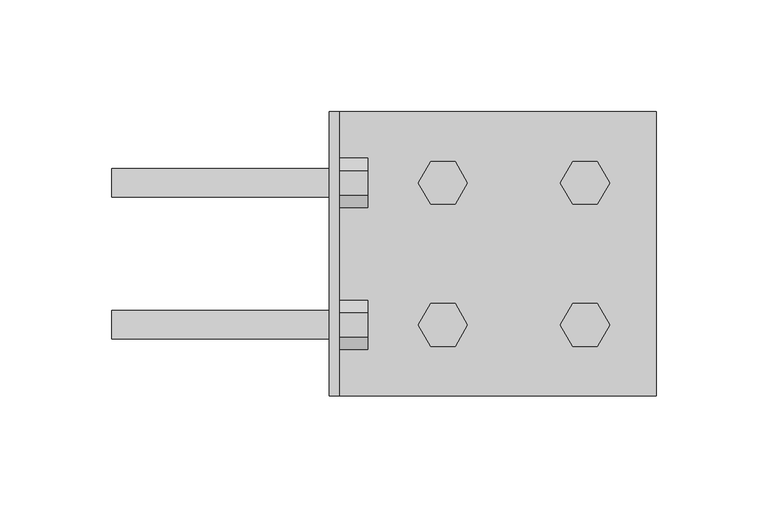
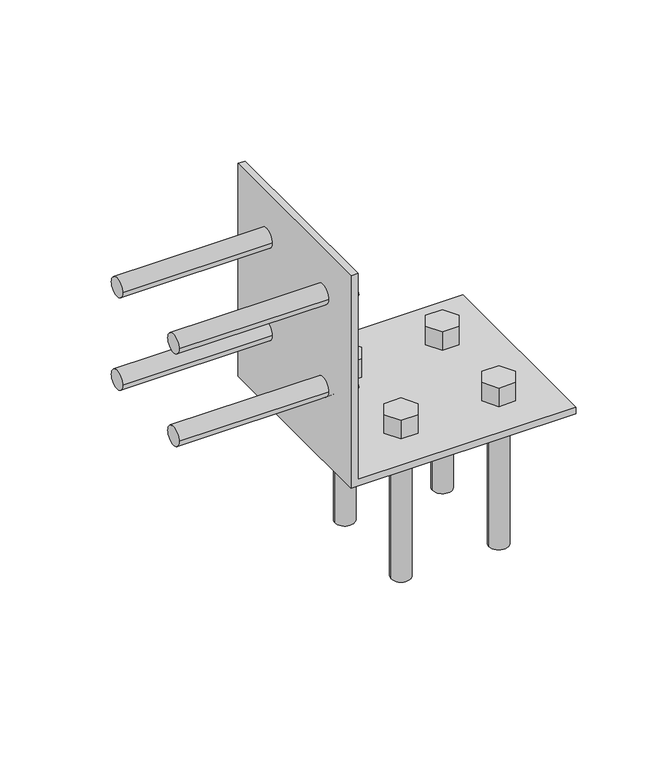
"""IFC4 building model written with IfcOpenShell, lengths in millimetres: fastener geometry."""

from ifc_helpers import new_model, si_unit, point, frame, frame_2d, origin, place, context, project, spatial, polyline, circle_curve, trimmed, segment, composite_curve, outline, extrude, source, transform, mapped, element, save
from ifc_brep_helpers import plane_surface, revolved_surface, advanced_brep


def fastener_5634bf7e(model_context):
    return source(origin(), model_context, "Body", "SolidModel", [
        extrude(outline(composite_curve([segment(trimmed(circle_curve(frame_2d((-31.75, 50.8)), 6.35), [point((-38.1, 50.8))], [point((-25.4, 50.8))], False, "CARTESIAN"), True, "CONTINUOUS"), segment(trimmed(circle_curve(frame_2d((-31.75, 50.8)), 6.35), [point((-25.4, 50.8))], [point((-38.1, 50.8))], False, "CARTESIAN"), True, "CONTINUOUS")], self_intersect=False)), frame((-97.0359375, 0.0, 0.0), z_axis=(1.0, 0.0, 0.0), x_axis=(0.0, 1.0, 0.0)), (0.0, 0.0, 1.0), 101.6),
        extrude(outline(polyline([(-42.7485226, 50.8), (-37.2492613, 60.325), (-26.2507387, 60.325), (-20.7514774, 50.8), (-26.2507387, 41.275), (-37.2492613, 41.275), (-42.7485226, 50.8)])), frame((4.5640625, 0.0, 0.0), z_axis=(1.0, 0.0, 0.0), x_axis=(0.0, 1.0, 0.0)), (0.0, 0.0, 1.0), 12.7),
        extrude(outline(composite_curve([segment(trimmed(circle_curve(frame_2d((31.75, 50.8)), 6.35), [point((25.4, 50.8))], [point((38.1, 50.8))], False, "CARTESIAN"), True, "CONTINUOUS"), segment(trimmed(circle_curve(frame_2d((31.75, 50.8)), 6.35), [point((38.1, 50.8))], [point((25.4, 50.8))], False, "CARTESIAN"), True, "CONTINUOUS")], self_intersect=False)), frame((-97.0359375, 0.0, 0.0), z_axis=(1.0, 0.0, 0.0), x_axis=(0.0, 1.0, 0.0)), (0.0, 0.0, 1.0), 101.6),
        extrude(outline(polyline([(20.7514774, 50.8), (26.2507387, 60.325), (37.2492613, 60.325), (42.7485226, 50.8), (37.2492613, 41.275), (26.2507387, 41.275), (20.7514774, 50.8)])), frame((4.5640625, 0.0, 0.0), z_axis=(1.0, 0.0, 0.0), x_axis=(0.0, 1.0, 0.0)), (0.0, 0.0, 1.0), 12.7),
        extrude(outline(composite_curve([segment(trimmed(circle_curve(frame_2d((31.75, 114.3)), 6.35), [point((25.4, 114.3))], [point((38.1, 114.3))], False, "CARTESIAN"), True, "CONTINUOUS"), segment(trimmed(circle_curve(frame_2d((31.75, 114.3)), 6.35), [point((38.1, 114.3))], [point((25.4, 114.3))], False, "CARTESIAN"), True, "CONTINUOUS")], self_intersect=False)), frame((-97.0359375, 0.0, 0.0), z_axis=(1.0, 0.0, 0.0), x_axis=(0.0, 1.0, 0.0)), (0.0, 0.0, 1.0), 101.6),
        extrude(outline(polyline([(20.7514774, 114.3), (26.2507387, 123.825), (37.2492613, 123.825), (42.7485226, 114.3), (37.2492613, 104.775), (26.2507387, 104.775), (20.7514774, 114.3)])), frame((4.5640625, 0.0, 0.0), z_axis=(1.0, 0.0, 0.0), x_axis=(0.0, 1.0, 0.0)), (0.0, 0.0, 1.0), 12.7),
        extrude(outline(composite_curve([segment(trimmed(circle_curve(frame_2d((-31.75, 114.3)), 6.35), [point((-38.1, 114.3))], [point((-25.4, 114.3))], False, "CARTESIAN"), True, "CONTINUOUS"), segment(trimmed(circle_curve(frame_2d((-31.75, 114.3)), 6.35), [point((-25.4, 114.3))], [point((-38.1, 114.3))], False, "CARTESIAN"), True, "CONTINUOUS")], self_intersect=False)), frame((-97.0359375, 0.0, 0.0), z_axis=(1.0, 0.0, 0.0), x_axis=(0.0, 1.0, 0.0)), (0.0, 0.0, 1.0), 101.6),
        extrude(outline(polyline([(-42.7485226, 114.3), (-37.2492613, 123.825), (-26.2507387, 123.825), (-20.7514774, 114.3), (-26.2507387, 104.775), (-37.2492613, 104.775), (-42.7485226, 114.3)])), frame((4.5640625, 0.0, 0.0), z_axis=(1.0, 0.0, 0.0), x_axis=(0.0, 1.0, 0.0)), (0.0, 0.0, 1.0), 12.7),
        extrude(outline(composite_curve([segment(trimmed(circle_curve(frame_2d((50.8, 31.75)), 6.35), [point((44.45, 31.75))], [point((57.15, 31.75))], False, "CARTESIAN"), True, "CONTINUOUS"), segment(trimmed(circle_curve(frame_2d((50.8, 31.75)), 6.35), [point((57.15, 31.75))], [point((44.45, 31.75))], False, "CARTESIAN"), True, "CONTINUOUS")], self_intersect=False)), frame((0.0, 0.0, -97.0359375), z_axis=(0.0, 0.0, 1.0), x_axis=(1.0, 0.0, 0.0)), (0.0, 0.0, 1.0), 101.6),
        extrude(outline(polyline([(39.8014774, 31.75), (45.3007387, 41.275), (56.2992613, 41.275), (61.7985226, 31.75), (56.2992613, 22.225), (45.3007387, 22.225), (39.8014774, 31.75)])), frame((0.0, 0.0, 4.5640625), z_axis=(0.0, 0.0, 1.0), x_axis=(1.0, 0.0, 0.0)), (0.0, 0.0, 1.0), 12.7),
        extrude(outline(composite_curve([segment(trimmed(circle_curve(frame_2d((114.3, 31.75)), 6.35), [point((107.95, 31.75))], [point((120.65, 31.75))], False, "CARTESIAN"), True, "CONTINUOUS"), segment(trimmed(circle_curve(frame_2d((114.3, 31.75)), 6.35), [point((120.65, 31.75))], [point((107.95, 31.75))], False, "CARTESIAN"), True, "CONTINUOUS")], self_intersect=False)), frame((0.0, 0.0, -97.0359375), z_axis=(0.0, 0.0, 1.0), x_axis=(1.0, 0.0, 0.0)), (0.0, 0.0, 1.0), 101.6),
        extrude(outline(polyline([(103.3014774, 31.75), (108.8007387, 41.275), (119.7992613, 41.275), (125.2985226, 31.75), (119.7992613, 22.225), (108.8007387, 22.225), (103.3014774, 31.75)])), frame((0.0, 0.0, 4.5640625), z_axis=(0.0, 0.0, 1.0), x_axis=(1.0, 0.0, 0.0)), (0.0, 0.0, 1.0), 12.7),
        extrude(outline(composite_curve([segment(trimmed(circle_curve(frame_2d((114.3, -31.75)), 6.35), [point((107.95, -31.75))], [point((120.65, -31.75))], False, "CARTESIAN"), True, "CONTINUOUS"), segment(trimmed(circle_curve(frame_2d((114.3, -31.75)), 6.35), [point((120.65, -31.75))], [point((107.95, -31.75))], False, "CARTESIAN"), True, "CONTINUOUS")], self_intersect=False)), frame((0.0, 0.0, -97.0359375), z_axis=(0.0, 0.0, 1.0), x_axis=(1.0, 0.0, 0.0)), (0.0, 0.0, 1.0), 101.6),
        extrude(outline(polyline([(103.3014774, -31.75), (108.8007387, -22.225), (119.7992613, -22.225), (125.2985226, -31.75), (119.7992613, -41.275), (108.8007387, -41.275), (103.3014774, -31.75)])), frame((0.0, 0.0, 4.5640625), z_axis=(0.0, 0.0, 1.0), x_axis=(1.0, 0.0, 0.0)), (0.0, 0.0, 1.0), 12.7),
        extrude(outline(composite_curve([segment(trimmed(circle_curve(frame_2d((50.8, -31.75)), 6.35), [point((44.45, -31.75))], [point((57.15, -31.75))], False, "CARTESIAN"), True, "CONTINUOUS"), segment(trimmed(circle_curve(frame_2d((50.8, -31.75)), 6.35), [point((57.15, -31.75))], [point((44.45, -31.75))], False, "CARTESIAN"), True, "CONTINUOUS")], self_intersect=False)), frame((0.0, 0.0, -97.0359375), z_axis=(0.0, 0.0, 1.0), x_axis=(1.0, 0.0, 0.0)), (0.0, 0.0, 1.0), 101.6),
        extrude(outline(polyline([(39.8014774, -31.75), (45.3007387, -22.225), (56.2992613, -22.225), (61.7985226, -31.75), (56.2992613, -41.275), (45.3007387, -41.275), (39.8014774, -31.75)])), frame((0.0, 0.0, 4.5640625), z_axis=(0.0, 0.0, 1.0), x_axis=(1.0, 0.0, 0.0)), (0.0, 0.0, 1.0), 12.7),
        advanced_brep(
        [(4.5640625, 63.5, 146.05), (4.5640625, -63.5, 146.05), (4.5640625, -63.5, 4.5640625), (4.5640625, 63.5, 4.5640625), (4.5640625, -25.4, 50.8), (4.5640625, -38.1, 50.8), (4.5640625, 38.1, 50.8), (4.5640625, 25.4, 50.8), (4.5640625, 38.1, 114.3), (4.5640625, 25.4, 114.3), (4.5640625, -25.4, 114.3), (4.5640625, -38.1, 114.3), (0.0, -63.5, 146.05), (0.0, 63.5, 146.05), (0.0, 63.5, 0.0), (0.0, -63.5, 0.0), (0.0, -38.1, 50.8), (0.0, -25.4, 50.8), (0.0, 25.4, 50.8), (0.0, 38.1, 50.8), (0.0, 25.4, 114.3), (0.0, 38.1, 114.3), (0.0, -38.1, 114.3), (0.0, -25.4, 114.3), (146.05, -63.5, 0.0), (146.05, -63.5, 4.5640625), (146.05, 63.5, 4.5640625), (146.05, 63.5, 0.0), (57.15, -31.75, 4.5640625), (44.45, -31.75, 4.5640625), (120.65, -31.75, 4.5640625), (107.95, -31.75, 4.5640625), (57.15, 31.75, 4.5640625), (44.45, 31.75, 4.5640625), (120.65, 31.75, 4.5640625), (107.95, 31.75, 4.5640625), (44.45, -31.75, 0.0), (57.15, -31.75, 0.0), (107.95, -31.75, 0.0), (120.65, -31.75, 0.0), (44.45, 31.75, 0.0), (57.15, 31.75, 0.0), (107.95, 31.75, 0.0), (120.65, 31.75, 0.0)],
        [
            (0, 1),
            (1, 2),
            (2, 3),
            (3, 0),
            (4, 5, circle_curve(frame((4.5640625, -31.75, 50.8), z_axis=(-1.0, 0.0, 0.0), x_axis=(0.0, 1.0, 0.0)), 6.35)),
            (5, 4, circle_curve(frame((4.5640625, -31.75, 50.8), z_axis=(-1.0, 0.0, 0.0), x_axis=(0.0, 1.0, 0.0)), 6.35)),
            (6, 7, circle_curve(frame((4.5640625, 31.75, 50.8), z_axis=(-1.0, 0.0, 0.0), x_axis=(0.0, 1.0, 0.0)), 6.35)),
            (7, 6, circle_curve(frame((4.5640625, 31.75, 50.8), z_axis=(-1.0, 0.0, 0.0), x_axis=(0.0, 1.0, 0.0)), 6.35)),
            (8, 9, circle_curve(frame((4.5640625, 31.75, 114.3), z_axis=(-1.0, 0.0, 0.0), x_axis=(0.0, 1.0, 0.0)), 6.35)),
            (9, 8, circle_curve(frame((4.5640625, 31.75, 114.3), z_axis=(-1.0, 0.0, 0.0), x_axis=(0.0, 1.0, 0.0)), 6.35)),
            (10, 11, circle_curve(frame((4.5640625, -31.75, 114.3), z_axis=(-1.0, 0.0, 0.0), x_axis=(0.0, 1.0, 0.0)), 6.35)),
            (11, 10, circle_curve(frame((4.5640625, -31.75, 114.3), z_axis=(-1.0, 0.0, 0.0), x_axis=(0.0, 1.0, 0.0)), 6.35)),
            (12, 13),
            (13, 14),
            (14, 15),
            (15, 12),
            (16, 17, circle_curve(frame((0.0, -31.75, 50.8), z_axis=(1.0, 0.0, 0.0), x_axis=(0.0, 1.0, 0.0)), 6.35)),
            (17, 16, circle_curve(frame((0.0, -31.75, 50.8), z_axis=(1.0, 0.0, 0.0), x_axis=(0.0, 1.0, 0.0)), 6.35)),
            (18, 19, circle_curve(frame((0.0, 31.75, 50.8), z_axis=(1.0, 0.0, 0.0), x_axis=(0.0, 1.0, 0.0)), 6.35)),
            (19, 18, circle_curve(frame((0.0, 31.75, 50.8), z_axis=(1.0, 0.0, 0.0), x_axis=(0.0, 1.0, 0.0)), 6.35)),
            (20, 21, circle_curve(frame((0.0, 31.75, 114.3), z_axis=(1.0, 0.0, 0.0), x_axis=(0.0, 1.0, 0.0)), 6.35)),
            (21, 20, circle_curve(frame((0.0, 31.75, 114.3), z_axis=(1.0, 0.0, 0.0), x_axis=(0.0, 1.0, 0.0)), 6.35)),
            (22, 23, circle_curve(frame((0.0, -31.75, 114.3), z_axis=(1.0, 0.0, 0.0), x_axis=(0.0, 1.0, 0.0)), 6.35)),
            (23, 22, circle_curve(frame((0.0, -31.75, 114.3), z_axis=(1.0, 0.0, 0.0), x_axis=(0.0, 1.0, 0.0)), 6.35)),
            (0, 13),
            (12, 1),
            (15, 24),
            (24, 25),
            (25, 2),
            (3, 26),
            (26, 27),
            (27, 14),
            (25, 26),
            (28, 29, circle_curve(frame((50.8, -31.75, 4.5640625), z_axis=(0.0, 0.0, -1.0), x_axis=(1.0, 0.0, 0.0)), 6.35)),
            (29, 28, circle_curve(frame((50.8, -31.75, 4.5640625), z_axis=(0.0, 0.0, -1.0), x_axis=(1.0, 0.0, 0.0)), 6.35)),
            (30, 31, circle_curve(frame((114.3, -31.75, 4.5640625), z_axis=(0.0, 0.0, -1.0), x_axis=(1.0, 0.0, 0.0)), 6.35)),
            (31, 30, circle_curve(frame((114.3, -31.75, 4.5640625), z_axis=(0.0, 0.0, -1.0), x_axis=(1.0, 0.0, 0.0)), 6.35)),
            (32, 33, circle_curve(frame((50.8, 31.75, 4.5640625), z_axis=(0.0, 0.0, -1.0), x_axis=(1.0, 0.0, 0.0)), 6.35)),
            (33, 32, circle_curve(frame((50.8, 31.75, 4.5640625), z_axis=(0.0, 0.0, -1.0), x_axis=(1.0, 0.0, 0.0)), 6.35)),
            (34, 35, circle_curve(frame((114.3, 31.75, 4.5640625), z_axis=(0.0, 0.0, -1.0), x_axis=(1.0, 0.0, 0.0)), 6.35)),
            (35, 34, circle_curve(frame((114.3, 31.75, 4.5640625), z_axis=(0.0, 0.0, -1.0), x_axis=(1.0, 0.0, 0.0)), 6.35)),
            (27, 24),
            (36, 37, circle_curve(frame((50.8, -31.75, 0.0), z_axis=(0.0, 0.0, 1.0), x_axis=(1.0, 0.0, 0.0)), 6.35)),
            (37, 36, circle_curve(frame((50.8, -31.75, 0.0), z_axis=(0.0, 0.0, 1.0), x_axis=(1.0, 0.0, 0.0)), 6.35)),
            (38, 39, circle_curve(frame((114.3, -31.75, 0.0), z_axis=(0.0, 0.0, 1.0), x_axis=(1.0, 0.0, 0.0)), 6.35)),
            (39, 38, circle_curve(frame((114.3, -31.75, 0.0), z_axis=(0.0, 0.0, 1.0), x_axis=(1.0, 0.0, 0.0)), 6.35)),
            (40, 41, circle_curve(frame((50.8, 31.75, 0.0), z_axis=(0.0, 0.0, 1.0), x_axis=(1.0, 0.0, 0.0)), 6.35)),
            (41, 40, circle_curve(frame((50.8, 31.75, 0.0), z_axis=(0.0, 0.0, 1.0), x_axis=(1.0, 0.0, 0.0)), 6.35)),
            (42, 43, circle_curve(frame((114.3, 31.75, 0.0), z_axis=(0.0, 0.0, 1.0), x_axis=(1.0, 0.0, 0.0)), 6.35)),
            (43, 42, circle_curve(frame((114.3, 31.75, 0.0), z_axis=(0.0, 0.0, 1.0), x_axis=(1.0, 0.0, 0.0)), 6.35)),
            (28, 37),
            (36, 29),
            (38, 31),
            (30, 39),
            (40, 33),
            (32, 41),
            (42, 35),
            (34, 43),
            (4, 17),
            (16, 5),
            (18, 7),
            (6, 19),
            (20, 9),
            (8, 21),
            (22, 11),
            (10, 23),
        ],
        [
            plane_surface(frame((4.5640625, -63.5, 146.05), z_axis=(1.0, 0.0, 0.0), x_axis=(0.0, -1.0, 0.0))),
            plane_surface(frame((0.0, -63.5, 146.05), z_axis=(-1.0, 0.0, 0.0), x_axis=(0.0, 1.0, 0.0))),
            plane_surface(frame((4.5640625, 63.5, 146.05), z_axis=(0.0, 0.0, 1.0), x_axis=(-1.0, 0.0, 0.0))),
            plane_surface(frame((4.5640625, -63.5, 146.05), z_axis=(0.0, -1.0, 0.0), x_axis=(-1.0, 0.0, 0.0))),
            plane_surface(frame((4.5640625, 63.5, 4.5640625), z_axis=(0.0, 1.0, 0.0), x_axis=(-1.0, 0.0, 0.0))),
            plane_surface(frame((0.0, 63.5, 4.5640625), z_axis=(0.0, 0.0, 1.0), x_axis=(-1.0, 0.0, 0.0))),
            plane_surface(frame((0.0, 63.5, 0.0), z_axis=(0.0, 0.0, -1.0), x_axis=(1.0, 0.0, 0.0))),
            plane_surface(frame((146.05, -63.5, 4.5640625), z_axis=(1.0, 0.0, 0.0), x_axis=(0.0, 0.0, -1.0))),
            revolved_surface(polyline([(57.15, -31.75, 4.5640625), (57.15, -31.75, 0.0)]), (50.8, -31.75, 0.0), (0.0, 0.0, 1.0)),
            revolved_surface(polyline([(120.64999999999999, -31.75, 4.5640625), (120.64999999999999, -31.75, 0.0)]), (114.3, -31.75, 0.0), (0.0, 0.0, 1.0)),
            revolved_surface(polyline([(57.15, 31.75, 4.5640625), (57.15, 31.75, 0.0)]), (50.8, 31.75, 0.0), (0.0, 0.0, 1.0)),
            revolved_surface(polyline([(120.64999999999999, 31.75, 4.5640625), (120.64999999999999, 31.75, 0.0)]), (114.3, 31.75, 0.0), (0.0, 0.0, 1.0)),
            revolved_surface(polyline([(4.5640625, -25.4, 50.8), (0.0, -25.4, 50.8)]), (0.0, -31.75, 50.8), (1.0, 0.0, 0.0)),
            revolved_surface(polyline([(4.5640625, 38.1, 50.8), (0.0, 38.1, 50.8)]), (0.0, 31.75, 50.8), (1.0, 0.0, 0.0)),
            revolved_surface(polyline([(4.5640625, 38.1, 114.3), (0.0, 38.1, 114.3)]), (0.0, 31.75, 114.3), (1.0, 0.0, 0.0)),
            revolved_surface(polyline([(4.5640625, -25.4, 114.3), (0.0, -25.4, 114.3)]), (0.0, -31.75, 114.3), (1.0, 0.0, 0.0)),
        ],
        [
            (0, [[1, 2, 3, 4], [5, 6], [7, 8], [9, 10], [11, 12]]),
            (1, [[13, 14, 15, 16], [17, 18], [19, 20], [21, 22], [23, 24]]),
            (2, [[-1, 25, -13, 26]]),
            (3, [[-2, -26, -16, 27, 28, 29]]),
            (4, [[-4, 30, 31, 32, -14, -25]]),
            (5, [[33, -30, -3, -29], [34, 35], [36, 37], [38, 39], [40, 41]]),
            (6, [[42, -27, -15, -32], [43, 44], [45, 46], [47, 48], [49, 50]]),
            (7, [[-33, -28, -42, -31]]),
            (8, [[51, -43, 52, -34]]),
            (8, [[-51, -35, -52, -44]]),
            (9, [[53, -36, 54, -45]]),
            (9, [[-53, -46, -54, -37]]),
            (10, [[55, -38, 56, -47]]),
            (10, [[-55, -48, -56, -39]]),
            (11, [[57, -40, 58, -49]]),
            (11, [[-57, -50, -58, -41]]),
            (12, [[59, -17, 60, -5]]),
            (12, [[-59, -6, -60, -18]]),
            (13, [[61, -7, 62, -19]]),
            (13, [[-61, -20, -62, -8]]),
            (14, [[63, -9, 64, -21]]),
            (14, [[-63, -22, -64, -10]]),
            (15, [[65, -11, 66, -23]]),
            (15, [[-65, -24, -66, -12]]),
        ],
    ),
    ])


if __name__ == "__main__":
    model = new_model("IFC4")
    model_context = context("Model", 3, world=origin())
    ifc_project = project(units=[si_unit("LENGTHUNIT", "METRE", prefix="MILLI")], contexts=[model_context])
    site = spatial("IfcSite", under=ifc_project)
    building = spatial("IfcBuilding", under=site)
    placement = place(None, origin())
    fastener_shape = fastener_5634bf7e(model_context)
    element("IfcFastener", 1, ObjectType="SIMPSON - HLPC/HLGPC Heavy Angles and Gussets : SIMPSON -HL55 - 5 X 5.75 - .5\" BOLT - HDG", at=placement, inside=building, context=model_context, shape_type="MappedRepresentation", body=[
        mapped(fastener_shape, transform((0.0, 0.0, 0.0), x_axis=(1.0, 0.0, 0.0), y_axis=(0.0, 1.0, 0.0), z_axis=(0.0, 0.0, 1.0))),
    ])
    save(model, "model.ifc")

# Revit data of these elements
# Type "SIMPSON - HLPC/HLGPC Heavy Angles and Gussets : SIMPSON -HL55 - 5 X 5.75 - .5\" BOLT - HDG"
#   URL = "https://www.strongtie.com/classiccollection_architecturalproductsgroup/hlpc-hlgpc_productgroup_wcc/p/hlpc.hlgpc"
#   L = 0' - 5"
#   Hole Radius = 0' - 0 1/4"
#   D4 = 0' - 2 1/2"
#   D2 = 0' - 2 1/2"
#   D1 = 0' - 1 1/4"
#   D3 = 0' - 2"
#   Ga. = 0' - 0 23/128"
#   W1 & W2 = 0' - 5 3/4"
#   Default Elevation = 4' - 0"
#   Bolt Visibility - 3B = no
#   Bolt Visibility - 3A = no
#   Bolt Visibility - 2B = yes
#   Bolt Visibility - 2A = yes
#   Bolt Visibility - 1B = yes
#   Bolt Visibility - 1A = yes
#   Bolt Visibility = yes
#   Bolt Size = element 1298416
# Element 1 (IfcFastener, "SIMPSON - HLPC/HLGPC Heavy Angles and Gussets : SIMPSON -HL55 - 5 X 5.75 - .5\" BOLT - HDG")
#   Materials on its faces: "1/2\" X 5\" LAG BOLT (THRU BOLT IF PLATE ON OPP. SIDE OF STRUCT MEMBER)"
# Materials
#   "1/2\" X 5\" LAG BOLT (THRU BOLT IF PLATE ON OPP. SIDE OF STRUCT MEMBER)": class "Generic", colour RGB 120 120 120, transparency 0, Cost = 0
